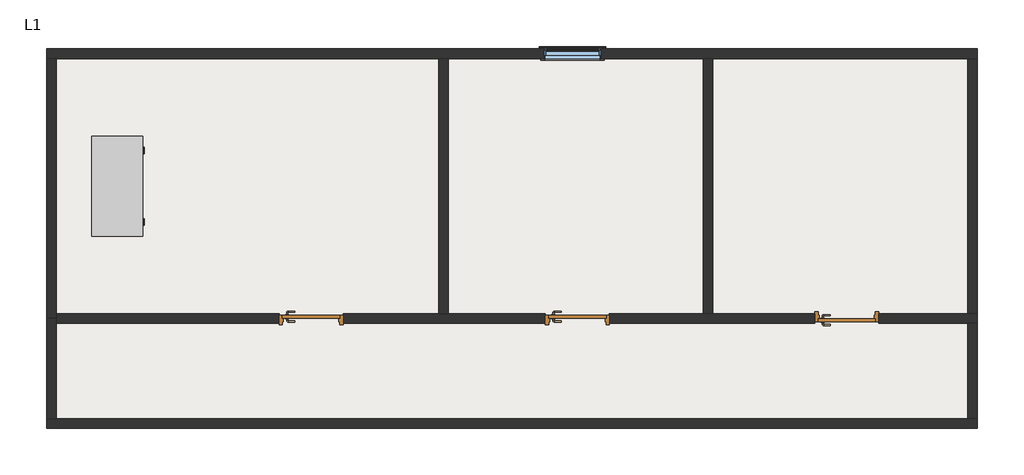
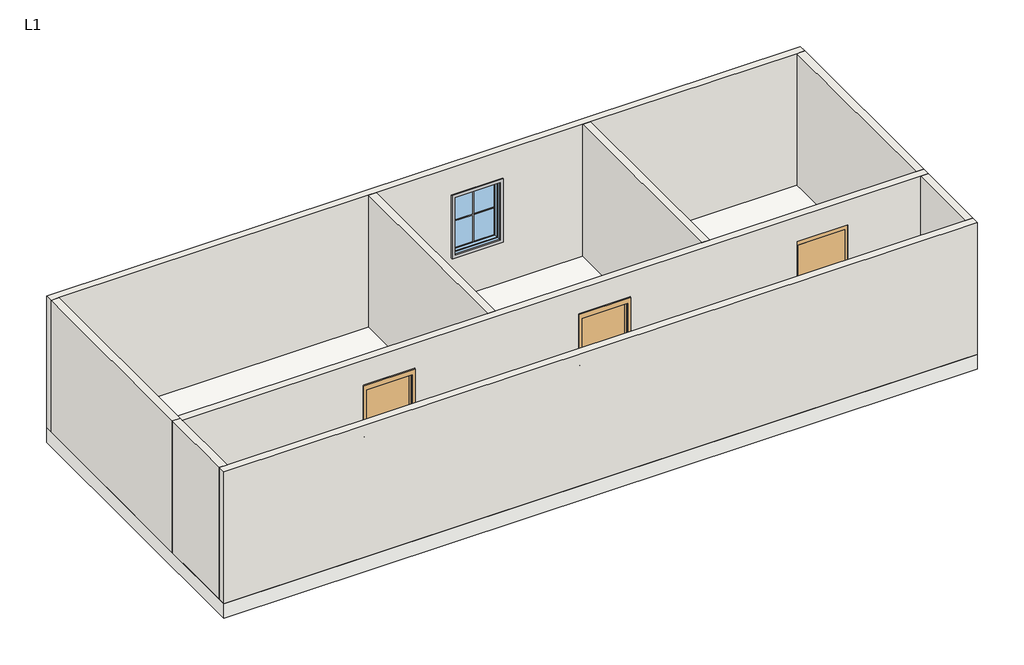
# One storey: 9 walls, 3 doors, 3 proxies, 1 furniture element, 1 slab, 1 window.
# Revit data of these elements (continued)
# Type "M_Muntin Pattern_2x2 : M_Muntin Pattern_2x2" (continued)
#   Width [instance default] = 1200 mm
#   Thickness = 12.7 mm
#   Height [instance default] = 1200 mm
#   Distance = 19.05 mm
#   Interior Material [instance default] = none
#   Exterior Material [instance default] = none
#   Default Elevation = 0
# Type "M_Trim-Window-Exterior-Flat : with Sill"
#   Trim Width = 60 mm
#   Trim Thickness_Picture Frame = 30 mm
#   Trim Thickness_with Sill = 19.05 mm
#   Sill Thickness = 30 mm
#   Opening Width [instance default] = 600 mm
#   Opening Height [instance default] = 900 mm
#   Default Elevation = 1200 mm
#   Sill = yes
#   Picture Frame = no
#   Trim Material [instance default] = none
# Type "M_Trim-Window-Interior-Flat : Picture Frame"
#   Trim Thickness_Picture Frame = 30 mm
#   Trim Width = 60 mm
#   Trim Thickness_with Sill = 20 mm
#   Sill Thickness = 30 mm
#   Opening Width [instance default] = 600 mm
#   Opening Height [instance default] = 900 mm
#   Default Elevation = 1200 mm
#   Sill = no
#   Picture Frame = yes
#   Trim Material [instance default] = none
# Type "M_Door-Passage-Single-Flush : 900 x 2100mm"
#   Type Mark = "38"
#   Analytic Construction = "Wooden"
#   Thickness = 45 mm
#   Thermal Resistance (R) = 0.455703 (m²·K)/W
#   Swing Angle [instance default] = 90.00°
#   Strike Height = 1000 mm
#   Rough Width [instance default] = 1000 mm
#   Rough Height [instance default] = 2200 mm
#   MF Opening Height [instance default] = 100 mm
#   MF Opening Width [instance default] = 100 mm
#   Inset Calculate [instance default] = 105 mm
#   Masonry Inset [instance default] = 25 mm
#   Height = 2100 mm
#   Width = 900 mm
#   Heat Transfer Coefficient (U) = 2.19465 W/(m²·K)
#   Masonry Frame Depth = 150 mm
#   Masonry Frame [instance default] = yes
#   Function = 1
#   Dry Wall Frame [instance default] = no
#   Panel Material = Wood - Birch
#   Frame Material = Metal - Paint Finish - Grey
#   Door Handle Material = Aluminum
#   Visual Light Transmittance = 0
#   Solar Heat Gain Coefficient = 0
#   Wall Closure = (empty or 0)
# Type "M_Desk : 1525 x 762mm Student"
#   Depth = 762 mm
#   Height = 762 mm
#   Leg Height = 152 mm
#   Width = 1525 mm
#   Body Material = Laminate, Ivory, Matte
#   Handle/Leg Material = Steel, Chrome Plated
#   Top Material = Cherry
#   Default Elevation = 0
# Type "Generic 300mm"
#   Description = "Generic Floor (Material By Category), 300mm thick"
#   Function = 0
#   Layers, outside or top first: 300 mm no material (function 1)
# Type "Generic - 150mm"
#   Description = "Generic Wall (Material By Category), 150mm thick"
#   Type Mark = "G04"
#   Layers, outside or top first: 150 mm no material (function 1)
# Type "M_Window-Fixed : 900 x 1200mm"
#   Type Mark = "36"
#   Fire Rating = "0.5h"
#   Analytic Construction = "Double glazing - domestic"
#   Window Inset [instance default] = 0 mm
#   Wall Thickness [instance default] = 150 mm
#   Visual Light Transmittance = 0.81
#   Thermal Resistance (R) = 0.319569 (m²·K)/W
#   Solar Heat Gain Coefficient = 0.76
#   Rough Width = 915 mm
#   Rough Height = 1215 mm
#   Interior Wall Closure [instance default] = 54.75 mm
#   Height = 1200 mm
#   Heat Transfer Coefficient (U) = 3.12929 W/(m²·K)
#   Frame Extension [instance default] = 6.35 mm
#   Exterior Wall Closure [instance default] = 31.75 mm
#   Extension Jamb [instance default] = 54.75 mm
#   Default Sill Height = 900 mm
#   Width = 900 mm
#   Muntin Visibility = yes
#   Interior Trim Visibility [instance default] = yes
#   Exterior Trim Visibility [instance default] = yes
#   Extension Jamb Visibility [instance default] = yes
#   Muntin Pattern = M_Muntin Pattern_2x2 : M_Muntin Pattern_2x2
#   Interior Trim Material = Wood - Stained
#   Interior Trim = M_Trim-Window-Interior-Flat : Picture Frame
#   Interior Frame Material = Wood - Stained
#   Glass Panel Material = Glass
#   Exterior Trim Material = Clad - White
#   Exterior Trim = M_Trim-Window-Exterior-Flat : with Sill
#   Exterior Frame Material = Clad - White
#   Wall Closure = (empty or 0)
# Element 1 (IfcBuildingElementProxy, "M_Muntin Pattern_2x2 : M_Muntin Pattern_2x2")
#   Width = 823.8 mm
#   Height = 1123.8 mm
#   Interior Material = Wood - Stained
#   Exterior Material = Clad - White
#   Phase Created = New Construction
#   Materials on its faces: "Clad - White", "Wood - Stained"
# Element 2 (IfcBuildingElementProxy, "M_Trim-Window-Exterior-Flat : with Sill")
#   Opening Width = 900 mm
#   Opening Height = 1200 mm
#   Trim Material = Clad - White
#   Phase Created = New Construction
#   Materials on its faces: "Clad - White"
# Element 3 (IfcBuildingElementProxy, "M_Trim-Window-Interior-Flat : Picture Frame")
#   Opening Width = 900 mm
#   Opening Height = 1200 mm
#   Trim Material = Wood - Stained
#   Phase Created = New Construction
#   Materials on its faces: "Wood - Stained"
# Elements 4, 5, 6 (IfcDoor, "M_Door-Passage-Single-Flush : 900 x 2100mm")
#   Swing Angle = 90.00°
#   Rough Width = 1000 mm
#   Rough Height = 2200 mm
#   Masonry Inset = 25 mm
#   MF Opening Width = 100 mm
#   MF Opening Height = 100 mm
#   Inset Calculate = 105 mm
#   Masonry Frame = yes
#   Dry Wall Frame = no
#   Phase Created = New Construction
#   Materials on its faces: "Aluminum", "Metal - Paint Finish - Grey", "Wood - Birch"
# Element 7 (IfcFurniture, "M_Desk : 1525 x 762mm Student")
#   Phase Created = New Construction
#   Materials on its faces: "Steel, Chrome Plated", "Laminate, Ivory, Matte", "Cherry"
# Element 8 (IfcSlab, "Generic 300mm")
#   Height Offset From Level = 0 mm
#   Phase Created = New Construction
#   Materials on its faces: "Default Floor"
# Elements 9, 10, 11, 12, 13, 14, 15, 17 (IfcWall, "Generic - 150mm")
#   Top Offset = 0 mm
#   Base Offset = 0 mm
#   Unconnected Height = 2700 mm
#   wall height = 2700 mm
#   Phase Created = New Construction
#   Base Constraint = L1
#   Materials on its faces: "Default Wall"
# Element 16 (IfcWall, "Generic - 150mm")
#   Top Offset = 0 mm
#   Base Offset = 0 mm
#   wall height = 2700 mm
#   Phase Created = New Construction
#   Base Constraint = L1
#   Top Constraint = L2
#   Materials on its faces: "Default Wall"
# Element 18 (IfcWindow, "M_Window-Fixed : 900 x 1200mm")
#   Mark = "107"
#   Window Inset = 0 mm
#   Interior Wall Closure = 54.75 mm
#   Frame Extension = 6.35 mm
#   Exterior Wall Closure = 31.75 mm
#   Interior Trim Visibility = yes
#   Exterior Trim Visibility = yes
#   Phase Created = New Construction
#   Materials on its faces: "Wood - Stained", "Glass", "Clad - White"
# Materials
#   "Wood - Birch": class "Wood", colour RGB 173 132 96, transparency 0, Cost = 0
#   "Metal - Paint Finish - Grey": class "Paint", colour RGB 178 178 178, transparency 0, Cost = 0
#   "Aluminum": class "Metal", colour RGB 244 245 246, transparency 0, Description = "Aluminum 6061", Cost = 0
#   "Laminate, Ivory, Matte": class "Plastic", colour RGB 244 244 244, transparency 0, Description = "Plastic Laminate - Ivory, Matte", Cost = 0
#   "Steel, Chrome Plated": class "Metal", colour RGB 17 17 17, transparency 0, Description = "Chromiuim plated steel", Cost = 0
#   "Cherry": class "Wood", colour RGB 158 77 40, transparency 0, Description = "Prunus Serotina", Cost = 0
#   "Wood - Stained": class "Wood", colour RGB 173 132 96, transparency 0, Cost = 0
#   "Glass": class "Glass", colour RGB 245 245 243, transparency 1, Description = "Soda Lime Glass", Cost = 0
#   "Clad - White": class "Wood", colour RGB 245 245 243, transparency 0, Cost = 0
#   "Default Floor": class "Miscellaneous", colour RGB 128 128 128, transparency 0, Cost = 0
#   "Default Wall": class "Miscellaneous", colour RGB 192 192 192, transparency 0, Cost = 0
# Room at (2014.522, 2057.738) mm, phase "New Construction", upper level "L1", upper offset 3048 mm, lower offset 0 mm
#   Number = "100"
#   Name = "Room Name"
# Room at (-3400.268, 2057.738) mm, phase "New Construction", upper level "L1", upper offset 3048 mm, lower offset 0 mm
#   Number = "101"
#   Name = "Room Name"
# Room at (6134.471, 2057.738) mm, phase "New Construction", upper level "L1", upper offset 3048 mm, lower offset 0 mm
#   Number = "102"
#   Name = "Room Name"
# Room at (460.713, -885.082) mm, phase "New Construction", upper level "L1", upper offset 3048 mm, lower offset 0 mm
#   Number = "103"
#   Name = "Room Name"
